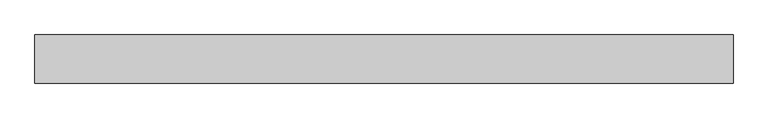
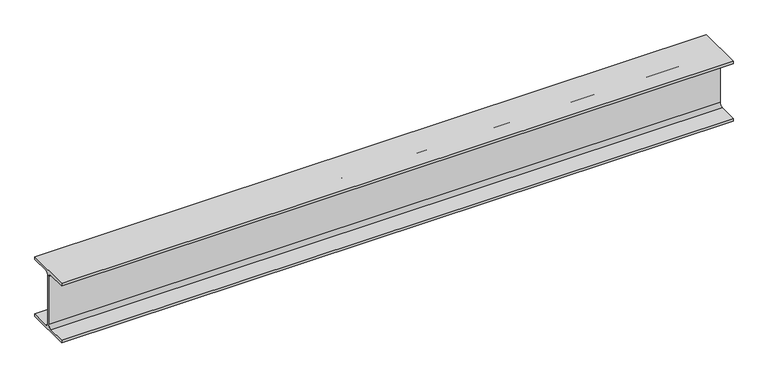
"""IFC4 building model written with IfcOpenShell, lengths in millimetres: beam geometry, 0912_Steel Framing_H-KSD3502 : H_SB_ASB_H-340x250x9x14."""

from ifc_helpers import new_model, si_unit, point, frame, frame_2d, origin, place, context, project, spatial, polyline, circle_curve, trimmed, segment, composite_curve, outline, extrude, source, transform, mapped, element, save


def beam_41a26c07(model_context):
    return source(origin(), model_context, "Body", "SweptSolid", [
        extrude(outline(composite_curve([segment(polyline([(125.0, -156.0), (125.0, -170.0), (-125.0, -170.0), (-125.0, -156.0), (-24.5, -156.0)]), True, "CONTINUOUS"), segment(trimmed(circle_curve(frame_2d((-24.5, -136.0)), 20.0), [point((-24.5, -156.0))], [point((-4.5, -136.0))], True, "CARTESIAN"), True, "CONTINUOUS"), segment(polyline([(-4.5, -136.0), (-4.5, 136.0)]), True, "CONTINUOUS"), segment(trimmed(circle_curve(frame_2d((-24.5, 136.0)), 20.0), [point((-4.5, 136.0))], [point((-24.5, 156.0))], True, "CARTESIAN"), True, "CONTINUOUS"), segment(polyline([(-24.5, 156.0), (-125.0, 156.0), (-125.0, 170.0), (125.0, 170.0), (125.0, 156.0), (24.5, 156.0)]), True, "CONTINUOUS"), segment(trimmed(circle_curve(frame_2d((24.5, 136.0)), 20.0), [point((24.5, 156.0))], [point((4.5, 136.0))], True, "CARTESIAN"), True, "CONTINUOUS"), segment(polyline([(4.5, 136.0), (4.5, -136.0)]), True, "CONTINUOUS"), segment(trimmed(circle_curve(frame_2d((24.5, -136.0)), 20.0), [point((4.5, -136.0))], [point((24.5, -156.0))], True, "CARTESIAN"), True, "CONTINUOUS"), segment(polyline([(24.5, -156.0), (125.0, -156.0)]), True, "CONTINUOUS")], self_intersect=False)), frame((-1812.3, 0.0, 0.0), z_axis=(1.0, 0.0, 0.0), x_axis=(0.0, 1.0, 0.0)), (0.0, 0.0, 1.0), 3624.6),
    ])


if __name__ == "__main__":
    model = new_model("IFC4")
    model_context = context("Model", 3, world=origin())
    ifc_project = project(units=[si_unit("LENGTHUNIT", "METRE", prefix="MILLI")], contexts=[model_context])
    site = spatial("IfcSite", under=ifc_project)
    building = spatial("IfcBuilding", under=site)
    placement = place(None, origin())
    beam_shape = beam_41a26c07(model_context)
    element("IfcBeam", 1, ObjectType="0912_Steel Framing_H-KSD3502 : H_SB_ASB_H-340x250x9x14", at=placement, inside=building, context=model_context, shape_type="MappedRepresentation", body=[
        mapped(beam_shape, transform((0.0, 0.0, 0.0), x_axis=(1.0, 0.0, 0.0), y_axis=(0.0, 1.0, 0.0), z_axis=(0.0, 0.0, 1.0))),
    ])
    save(model, "model.ifc")

# Revit data of these elements
# Type "0912_Steel Framing_H-KSD3502 : H_SB_ASB_H-340x250x9x14"
#   H_WM Code_1 = "S01AA002-00001 | Main Steel Structure Fabrication Work | Shelter/Building | Medium Steel - Standard (90KG/M>Weight≥30KG/M) | Material: (   )"
#   H_WM Code_2 = "S03AA028-00001 | Main Steel Structure Erection Work | Shelter/Building | Medium Steel (90KG/M>Weight≥30KG/M) | Material: (   )"
#   H_WM Code_3 = "S01AA010-00001 | Main Steel Structure Fabrication Work | Shelter/Building | Steel Painting/Coating | for Non-Fireproofed Steel Surface, Surface Preparation, Primer, Second & Final Coat | Material: (   )"
#   H_Q'ty Cal Type Tag = "SB-Q2"
#   Width = 25.0 cm
#   Web Thickness = 0.9 cm
#   Web Fillet = 2.0 cm
#   Warping Constant = 969000.0 cm⁶
#   W = 0
#   Torsional Moment of Inertia = 53.6551 cm⁴
#   Section Area = 101.5 cm²
#   Plastic Modulus weak axis = 447.0 cm³
#   Plastic Modulus strong axis = 1410.0 cm³
#   Perimeter = 1.63 m²/m
#   Nominal Weight = 79.70 kgf/m
#   Moment of Inertia weak axis = 3650.00 cm⁴
#   Moment of Inertia strong axis = 21700.00 cm⁴
#   Height = 34.0 cm
#   Flange Thickness = 1.4 cm
#   Elastic Modulus weak axis = 292.0 cm³
#   Elastic Modulus strong axis = 1280.0 cm³
#   Centroid Vertical = 17.0 cm
#   Centroid Horizontal = 12.5 cm
#   Ix = 217000000
#   Length [instance default] = 1.5240 m
#   Zx = 1410000
#   b = 0.2500 m
#   h = 0.3400 m
#   r = 0.0200 m
#   s = 0.0090 m
#   t = 0.0140 m
#   A = 0.01015 m²
#   Structural Material [instance default] = Steel, 45-345
#   Assembly Code = ""
# Element 1 (IfcBeam, "0912_Steel Framing_H-KSD3502 : H_SB_ASB_H-340x250x9x14")
#   Structural Material = none
# Materials
#   "Steel, 45-345": class "Metal", colour RGB 189 187 185, transparency 0, Description = "Steel 345 MPa", Cost = 0
